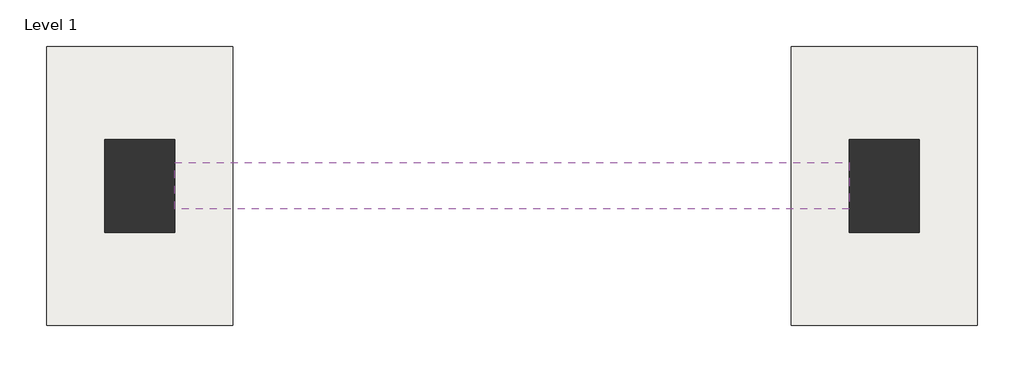
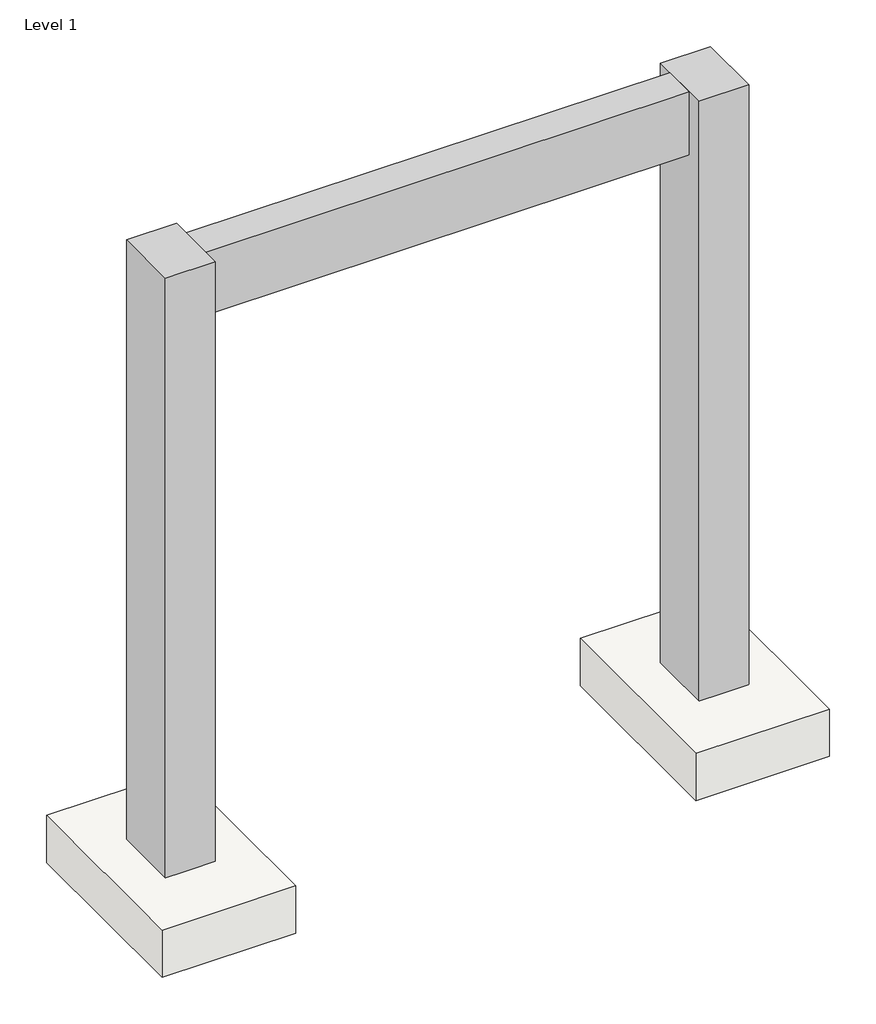
# One storey: 2 columns, 2 slabs, 1 beam.
"""IFC4 building model written with IfcOpenShell, lengths in millimetres."""

import ifcopenshell
import ifcopenshell.guid

model = None  # the IFC model being written
_history = None  # IfcOwnerHistory: only IFC2X3 demands one
_inside = {}  # id of a spatial element -> (the spatial element, [elements in it])
_under = {}  # id of a project, library or spatial element -> (it, [spatial elements below it])
_declared = {}  # id of a project -> (the project, [libraries it declares])
_typed = {}  # id of a type object -> (the type object, [elements of that type])
_made_of = {}  # id of a material, layer set ... -> (it, [elements and type objects made of it])


def new_model(schema):
    """Start an empty IFC model of exactly this schema.

    Asked for "IFC4X3", IfcOpenShell would pick the latest addendum, in which some entities
    have other attributes; the version numbers below select the first issue.
    IFC2X3 requires an IfcOwnerHistory on every rooted entity: one is made here for all.
    """
    global model, _history
    if schema == "IFC4X3":
        model = ifcopenshell.file(schema_version=(4, 3, 0, 0))
    else:
        model = ifcopenshell.file(schema=schema)
    _inside.clear()
    _under.clear()
    _declared.clear()
    _typed.clear()
    _made_of.clear()
    _history = None
    if model.schema == "IFC2X3":
        org = make("IfcOrganization", Name="unknown")
        user = make(
            "IfcPersonAndOrganization",
            ThePerson=make("IfcPerson", FamilyName="unknown"),
            TheOrganization=org,
        )
        app = make(
            "IfcApplication",
            ApplicationDeveloper=org,
            Version="unknown",
            ApplicationFullName="unknown",
            ApplicationIdentifier="unknown",
        )
        _history = make(
            "IfcOwnerHistory",
            OwningUser=user,
            OwningApplication=app,
            ChangeAction="ADDED",
            CreationDate=0,
        )
    return model


def make(cls, **values):
    """One entity of the class cls with the attributes given. An attribute that is None is left unset."""
    return model.create_entity(
        cls, **{name: value for name, value in values.items() if value is not None}
    )


def rooted(cls, **values):
    """An entity with a GlobalId (a new one), such as an element, a storey or a relation."""
    return make(cls, GlobalId=ifcopenshell.guid.new(), OwnerHistory=_history, **values)


def si_unit(unit_type, name, prefix=None):
    """IfcSIUnit, for example si_unit("LENGTHUNIT", "METRE", prefix="MILLI")."""
    return make("IfcSIUnit", UnitType=unit_type, Prefix=prefix, Name=name)


def assignment(units):
    """IfcUnitAssignment: the units of a project."""
    return None if units is None else make("IfcUnitAssignment", Units=units)


def point(xyz):
    """IfcCartesianPoint."""
    return None if xyz is None else make("IfcCartesianPoint", Coordinates=xyz)


def direction(xyz):
    """IfcDirection."""
    return None if xyz is None else make("IfcDirection", DirectionRatios=xyz)


def frame(location, z_axis=None, x_axis=None):
    """IfcAxis2Placement3D, a coordinate frame: its origin and axes. An axis left out is left unset."""
    return make(
        "IfcAxis2Placement3D",
        Location=point(location),
        Axis=direction(z_axis),
        RefDirection=direction(x_axis),
    )


def origin():
    """The frame at (0, 0, 0) with its axes left unset."""
    return frame((0.0, 0.0, 0.0))


def place(relative_to, where):
    """IfcLocalPlacement: puts the frame where relative to a parent placement (None: the world)."""
    return make(
        "IfcLocalPlacement", PlacementRelTo=relative_to, RelativePlacement=where
    )


def context(
    kind, dimensions, precision=None, world=None, true_north=None, identifier=None
):
    """IfcGeometricRepresentationContext, for example the 3D "Model" context."""
    return make(
        "IfcGeometricRepresentationContext",
        ContextIdentifier=identifier,
        ContextType=kind,
        CoordinateSpaceDimension=dimensions,
        Precision=precision,
        WorldCoordinateSystem=world,
        TrueNorth=true_north,
    )


def project(units=None, contexts=None):
    """IfcProject with its units and contexts."""
    return rooted(
        "IfcProject",
        Name="project",
        RepresentationContexts=contexts,
        UnitsInContext=assignment(units),
    )


def spatial(cls, under=None, at=None, **own):
    """A site, building, storey or space (cls), placed at a placement, below another one or the project."""
    s = rooted(cls, ObjectPlacement=at, **own)
    if under is not None:
        _under.setdefault(under.id(), (under, []))[1].append(s)
    return s


def polyline(points):
    """IfcPolyline through the points."""
    return make("IfcPolyline", Points=[point(p) for p in points])


def outline(outer, holes=None, kind="AREA"):
    """IfcArbitraryClosedProfileDef: a profile drawn as a closed curve; with holes, ...WithVoids."""
    if holes is None:
        return make("IfcArbitraryClosedProfileDef", ProfileType=kind, OuterCurve=outer)
    return make(
        "IfcArbitraryProfileDefWithVoids",
        ProfileType=kind,
        OuterCurve=outer,
        InnerCurves=holes,
    )


def extrude(swept, where, along, depth):
    """IfcExtrudedAreaSolid: the profile swept, set in the frame where, extruded along a direction by depth."""
    return make(
        "IfcExtrudedAreaSolid",
        SweptArea=swept,
        Position=where,
        ExtrudedDirection=direction(along),
        Depth=depth,
    )


def shape(context_of_items, identifier, shape_type, items):
    """IfcShapeRepresentation: the items that make up one representation, for example the "Body"."""
    return make(
        "IfcShapeRepresentation",
        ContextOfItems=context_of_items,
        RepresentationIdentifier=identifier,
        RepresentationType=shape_type,
        Items=items,
    )


def source(mapping_origin, context_of_items, identifier, shape_type, items):
    """IfcRepresentationMap: a shape defined once, which mapped items show again and again."""
    return make(
        "IfcRepresentationMap",
        MappingOrigin=mapping_origin,
        MappedRepresentation=shape(context_of_items, identifier, shape_type, items),
    )


def transform(
    local_origin,
    x_axis=None,
    y_axis=None,
    z_axis=None,
    scale=None,
    scale2=None,
    scale3=None,
    uniform=True,
):
    """IfcCartesianTransformationOperator3D, or its non-uniform kind. x_axis, y_axis, z_axis: its Axis1, 2, 3."""
    if uniform:
        return make(
            "IfcCartesianTransformationOperator3D",
            Axis1=direction(x_axis),
            Axis2=direction(y_axis),
            LocalOrigin=point(local_origin),
            Scale=scale,
            Axis3=direction(z_axis),
        )
    return make(
        "IfcCartesianTransformationOperator3DnonUniform",
        Axis1=direction(x_axis),
        Axis2=direction(y_axis),
        LocalOrigin=point(local_origin),
        Scale=scale,
        Axis3=direction(z_axis),
        Scale2=scale2,
        Scale3=scale3,
    )


def mapped(mapping_source, mapping_target):
    """IfcMappedItem: shows the shape of a source again, moved by a transform."""
    return make(
        "IfcMappedItem", MappingSource=mapping_source, MappingTarget=mapping_target
    )


def made_of(thing, what):
    """Note that an element or type object is made of a material, layer set ...; save() writes the relation."""
    if what is not None:
        _made_of.setdefault(what.id(), (what, []))[1].append(thing)
    return thing


def element(
    cls,
    number,
    at=None,
    inside=None,
    cuts=None,
    type_object=None,
    material=None,
    context=None,
    identifier="Body",
    shape_type=None,
    held_by="IfcProductDefinitionShape",
    body=None,
    shapes=None,
    **own,
):
    """One element of the class cls, such as IfcWall. Its Tag is "e" and its number.

    at: its placement. inside: the storey or other place that contains it. cuts: it is an
    opening in that element (IfcRelVoidsElement). A single representation is given by context,
    identifier, shape_type and body (its items); several are given by shapes. held_by: the class
    of the entity that holds the representations. save() writes the other relations.
    """
    e = rooted(cls, Tag="e%d" % number, ObjectPlacement=at, **own)
    if body is not None:
        shapes = [shape(context, identifier, shape_type, body)]
    if shapes is not None:
        e.Representation = make(held_by, Representations=shapes)
    if inside is not None:
        _inside.setdefault(inside.id(), (inside, []))[1].append(e)
    if cuts is not None:
        rooted(
            "IfcRelVoidsElement", RelatingBuildingElement=cuts, RelatedOpeningElement=e
        )
    if type_object is not None:
        _typed.setdefault(type_object.id(), (type_object, []))[1].append(e)
    return made_of(e, material)


def aggregate(whole, parts):
    """IfcRelAggregates: a whole, such as a stair, and the parts it consists of."""
    return rooted("IfcRelAggregates", RelatingObject=whole, RelatedObjects=parts)


def save(model, path):
    """Write the relations noted so far, then the file.

    IfcRelAggregates (storeys below a building ...), IfcRelContainedInSpatialStructure (elements
    in a storey), IfcRelDefinesByType, IfcRelAssociatesMaterial and IfcRelDeclares: one each for
    every whole, place, type object, material and project.
    """
    for whole, parts in _under.values():
        aggregate(whole, parts)
    for where, things in _inside.values():
        rooted(
            "IfcRelContainedInSpatialStructure",
            RelatedElements=things,
            RelatingStructure=where,
        )
    for kind, things in _typed.values():
        rooted("IfcRelDefinesByType", RelatedObjects=things, RelatingType=kind)
    for what, things in _made_of.values():
        rooted("IfcRelAssociatesMaterial", RelatedObjects=things, RelatingMaterial=what)
    for by, libraries in _declared.values():
        rooted("IfcRelDeclares", RelatingContext=by, RelatedDefinitions=libraries)
    model.write(path)


def slab_5ba74754(model_context):
    return source(origin(), model_context, "Body", "SweptSolid", [
        extrude(outline(polyline([(609.6, 914.4), (609.6, -914.4), (-609.6, -914.4), (-609.6, 914.4), (609.6, 914.4)])), frame((0.0, 0.0, -457.2), z_axis=(0.0, 0.0, 1.0), x_axis=(1.0, 0.0, 0.0)), (0.0, 0.0, 1.0), 457.2),
    ])


model = new_model("IFC4")

# Units and contexts
model_context = context("Model", 3, world=origin())
ifc_project = project(units=[si_unit("LENGTHUNIT", "METRE", prefix="MILLI")], contexts=[model_context])

# Site, building, storey
site = spatial("IfcSite", under=ifc_project)
building = spatial("IfcBuilding", under=site)
storey = spatial("IfcBuildingStorey", under=building, Name="Level 1", Elevation=0.0)

# Beam
placement = place(None, origin())
element("IfcBeam", 1, ObjectType="Concrete-Rectangular Beam : 12 x 24", at=placement, inside=storey, context=model_context, shape_type="SweptSolid", body=[
    extrude(outline(polyline([(-11045.0800525, 5786.0323826), (-11045.0800525, 6090.8323826), (-6625.4800525, 6090.8323826), (-6625.4800525, 5786.0323826), (-11045.0800525, 5786.0323826)])), frame((0.0, 0.0, 2438.4), z_axis=(0.0, 0.0, 1.0), x_axis=(1.0, 0.0, 0.0)), (0.0, 0.0, 1.0), 609.6),
])

# Columns
element("IfcColumn", 2, ObjectType="Concrete-Rectangular-Column : 18 x 24", at=placement, inside=storey, context=model_context, shape_type="SweptSolid", body=[
    extrude(outline(polyline([(-11045.0800525, 6243.2323826), (-11045.0800525, 5633.6323826), (-11502.2800525, 5633.6323826), (-11502.2800525, 6243.2323826), (-11045.0800525, 6243.2323826)])), frame((0.0, 0.0, -2743.2), z_axis=(0.0, 0.0, 1.0), x_axis=(1.0, 0.0, 0.0)), (0.0, 0.0, 1.0), 5791.2),
])
element("IfcColumn", 3, ObjectType="Concrete-Rectangular-Column : 18 x 24", at=placement, inside=storey, context=model_context, shape_type="SweptSolid", body=[
    extrude(outline(polyline([(-6168.2800525, 6243.2323826), (-6168.2800525, 5633.6323826), (-6625.4800525, 5633.6323826), (-6625.4800525, 6243.2323826), (-6168.2800525, 6243.2323826)])), frame((0.0, 0.0, -2743.2), z_axis=(0.0, 0.0, 1.0), x_axis=(1.0, 0.0, 0.0)), (0.0, 0.0, 1.0), 5791.2),
])

# Slabs
slab_shape = slab_5ba74754(model_context)
element("IfcSlab", 4, ObjectType="Footing-Rectangular : 72\" x 48\" x 18\"", at=placement, inside=storey, context=model_context, shape_type="MappedRepresentation", body=[
    mapped(slab_shape, transform((-11273.6800525, 5938.4323826, -2743.2), x_axis=(1.0, 0.0, 0.0), y_axis=(0.0, 1.0, 0.0), z_axis=(0.0, 0.0, 1.0))),
])
element("IfcSlab", 5, ObjectType="Footing-Rectangular : 72\" x 48\" x 18\"", at=placement, inside=storey, context=model_context, shape_type="MappedRepresentation", body=[
    mapped(slab_shape, transform((-6396.8800525, 5938.4323826, -2743.2), x_axis=(1.0, 0.0, 0.0), y_axis=(0.0, 1.0, 0.0), z_axis=(0.0, 0.0, 1.0))),
])

save(model, "model.ifc")

# Revit data of these elements
# Project information
#   IfcSite GUID = "0_uRv84q9BH8BmbsCmODV5"
#   IfcBuilding GUID = "0_uRv84q9BH8BmbsCmODV6"
#   IfcProject GUID = "0_uRv84q9BH8BmbsCmODV7"
#   Project Issue Date = "Issue Date"
#   Project Status = "Project Status"
#   Client Name = "Owner"
#   Project Address = "Enter address here"
#   Project Name = "Project Name"
#   Project Number = "Project Number"
# Grids (mm)
#   "1": line (9019.216, 5938.432) -> (-21563.036, 5938.432)
#   "2": line (-11273.68, -9686.145) -> (-11273.68, 17085.235)
#   "3": line (-6396.88, 17085.235) -> (-6396.88, -9686.145)
#   "4": line (3059.851, 3438.432) -> (-21143.609, 3438.432)
# Type "Concrete-Rectangular Beam : 12 x 24"
#   Assembly Code = "B10"
#   Length [instance default] = 1.524 m
#   b = 0.3048 m
#   h = 0.6096 m
#   Structural Material [instance default] = Concrete - Cast-in-Place Concrete
# Type "Concrete-Rectangular-Column : 18 x 24"
#   Assembly Code = "B10"
#   b = 0.4572 m
#   h = 0.6096 m
#   Structural Material [instance default] = Concrete - Cast-in-Place Concrete
# Type "Footing-Rectangular : 72\" x 48\" x 18\""
#   Assembly Code = "A1010100"
#   Width = 1.2192 m
#   Length = 1.8288 m
#   Thickness = 0.4572 m
#   Structural Material [instance default] = Concrete - Cast-in-Place Concrete
# Element 1 (IfcBeam, "Concrete-Rectangular Beam : 12 x 24")
#   IfcGUID = "3t$hXKBBT1XgsJcGm04jPr"
#   Comments = ""
#   Structural Material = Concrete - Cast-in-Place Concrete
#   Phase Created = New Construction
#   Materials on its faces: "Concrete - Cast-in-Place Concrete"
# Element 2 (IfcColumn, "Concrete-Rectangular-Column : 18 x 24")
#   IfcGUID = "01h4Zn8Tr79QLhlf3oc5We"
#   Structural Material = Concrete - Cast-in-Place Concrete
#   Phase Created = New Construction
#   Materials on its faces: "Concrete - Cast-in-Place Concrete"
# Element 3 (IfcColumn, "Concrete-Rectangular-Column : 18 x 24")
#   IfcGUID = "01h4Zn8Tr79QLhlf3oc4Vl"
#   Structural Material = Concrete - Cast-in-Place Concrete
#   Phase Created = New Construction
#   Materials on its faces: "Concrete - Cast-in-Place Concrete"
# Element 4 (IfcSlab, "Footing-Rectangular : 72\" x 48\" x 18\"")
#   IfcGUID = "3t$hXKBBT1XgsJcGm04jJz"
#   Structural Material = Concrete - Cast-in-Place Concrete
#   Phase Created = New Construction
#   Materials on its faces: "Concrete - Cast-in-Place Concrete"
# Element 5 (IfcSlab, "Footing-Rectangular : 72\" x 48\" x 18\"")
#   IfcGUID = "3t$hXKBBT1XgsJcGm04jTw"
#   Comments = ""
#   Structural Material = Concrete - Cast-in-Place Concrete
#   Phase Created = New Construction
#   Materials on its faces: "Concrete - Cast-in-Place Concrete"
# Materials
#   "Concrete - Cast-in-Place Concrete": class "Concrete", colour RGB 192 192 192, transparency 0
